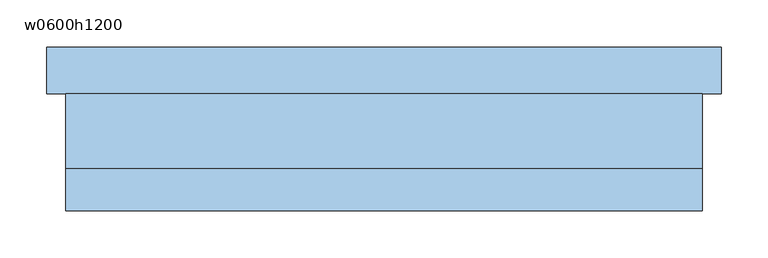
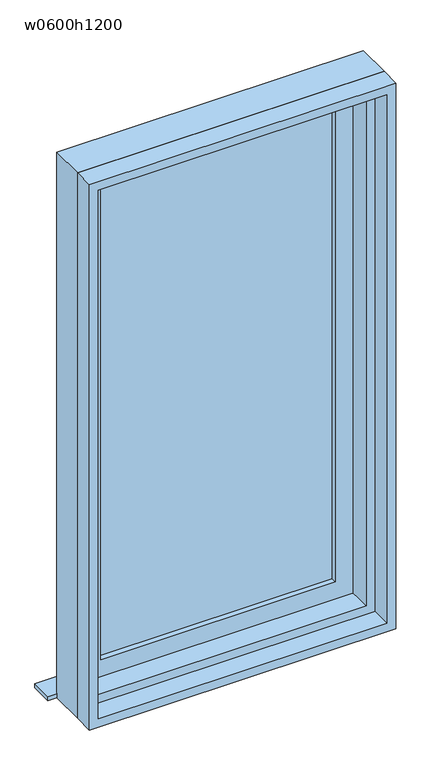
"""IFC4 building model written with IfcOpenShell, lengths in millimetres: window geometry, 縦すべり窓 : w0600h1200."""

import ifcopenshell
import ifcopenshell.guid

model = None  # the IFC model being written
_history = None  # IfcOwnerHistory: only IFC2X3 demands one
_inside = {}  # id of a spatial element -> (the spatial element, [elements in it])
_under = {}  # id of a project, library or spatial element -> (it, [spatial elements below it])
_declared = {}  # id of a project -> (the project, [libraries it declares])
_typed = {}  # id of a type object -> (the type object, [elements of that type])
_made_of = {}  # id of a material, layer set ... -> (it, [elements and type objects made of it])


def new_model(schema):
    """Start an empty IFC model of exactly this schema.

    Asked for "IFC4X3", IfcOpenShell would pick the latest addendum, in which some entities
    have other attributes; the version numbers below select the first issue.
    IFC2X3 requires an IfcOwnerHistory on every rooted entity: one is made here for all.
    """
    global model, _history
    if schema == "IFC4X3":
        model = ifcopenshell.file(schema_version=(4, 3, 0, 0))
    else:
        model = ifcopenshell.file(schema=schema)
    _inside.clear()
    _under.clear()
    _declared.clear()
    _typed.clear()
    _made_of.clear()
    _history = None
    if model.schema == "IFC2X3":
        org = make("IfcOrganization", Name="unknown")
        user = make(
            "IfcPersonAndOrganization",
            ThePerson=make("IfcPerson", FamilyName="unknown"),
            TheOrganization=org,
        )
        app = make(
            "IfcApplication",
            ApplicationDeveloper=org,
            Version="unknown",
            ApplicationFullName="unknown",
            ApplicationIdentifier="unknown",
        )
        _history = make(
            "IfcOwnerHistory",
            OwningUser=user,
            OwningApplication=app,
            ChangeAction="ADDED",
            CreationDate=0,
        )
    return model


def make(cls, **values):
    """One entity of the class cls with the attributes given. An attribute that is None is left unset."""
    return model.create_entity(
        cls, **{name: value for name, value in values.items() if value is not None}
    )


def rooted(cls, **values):
    """An entity with a GlobalId (a new one), such as an element, a storey or a relation."""
    return make(cls, GlobalId=ifcopenshell.guid.new(), OwnerHistory=_history, **values)


def si_unit(unit_type, name, prefix=None):
    """IfcSIUnit, for example si_unit("LENGTHUNIT", "METRE", prefix="MILLI")."""
    return make("IfcSIUnit", UnitType=unit_type, Prefix=prefix, Name=name)


def assignment(units):
    """IfcUnitAssignment: the units of a project."""
    return None if units is None else make("IfcUnitAssignment", Units=units)


def point(xyz):
    """IfcCartesianPoint."""
    return None if xyz is None else make("IfcCartesianPoint", Coordinates=xyz)


def direction(xyz):
    """IfcDirection."""
    return None if xyz is None else make("IfcDirection", DirectionRatios=xyz)


def frame(location, z_axis=None, x_axis=None):
    """IfcAxis2Placement3D, a coordinate frame: its origin and axes. An axis left out is left unset."""
    return make(
        "IfcAxis2Placement3D",
        Location=point(location),
        Axis=direction(z_axis),
        RefDirection=direction(x_axis),
    )


def origin():
    """The frame at (0, 0, 0) with its axes left unset."""
    return frame((0.0, 0.0, 0.0))


def place(relative_to, where):
    """IfcLocalPlacement: puts the frame where relative to a parent placement (None: the world)."""
    return make(
        "IfcLocalPlacement", PlacementRelTo=relative_to, RelativePlacement=where
    )


def context(
    kind, dimensions, precision=None, world=None, true_north=None, identifier=None
):
    """IfcGeometricRepresentationContext, for example the 3D "Model" context."""
    return make(
        "IfcGeometricRepresentationContext",
        ContextIdentifier=identifier,
        ContextType=kind,
        CoordinateSpaceDimension=dimensions,
        Precision=precision,
        WorldCoordinateSystem=world,
        TrueNorth=true_north,
    )


def project(units=None, contexts=None):
    """IfcProject with its units and contexts."""
    return rooted(
        "IfcProject",
        Name="project",
        RepresentationContexts=contexts,
        UnitsInContext=assignment(units),
    )


def spatial(cls, under=None, at=None, **own):
    """A site, building, storey or space (cls), placed at a placement, below another one or the project."""
    s = rooted(cls, ObjectPlacement=at, **own)
    if under is not None:
        _under.setdefault(under.id(), (under, []))[1].append(s)
    return s


def polyline(points):
    """IfcPolyline through the points."""
    return make("IfcPolyline", Points=[point(p) for p in points])


def outline(outer, holes=None, kind="AREA"):
    """IfcArbitraryClosedProfileDef: a profile drawn as a closed curve; with holes, ...WithVoids."""
    if holes is None:
        return make("IfcArbitraryClosedProfileDef", ProfileType=kind, OuterCurve=outer)
    return make(
        "IfcArbitraryProfileDefWithVoids",
        ProfileType=kind,
        OuterCurve=outer,
        InnerCurves=holes,
    )


def extrude(swept, where, along, depth):
    """IfcExtrudedAreaSolid: the profile swept, set in the frame where, extruded along a direction by depth."""
    return make(
        "IfcExtrudedAreaSolid",
        SweptArea=swept,
        Position=where,
        ExtrudedDirection=direction(along),
        Depth=depth,
    )


def shape(context_of_items, identifier, shape_type, items):
    """IfcShapeRepresentation: the items that make up one representation, for example the "Body"."""
    return make(
        "IfcShapeRepresentation",
        ContextOfItems=context_of_items,
        RepresentationIdentifier=identifier,
        RepresentationType=shape_type,
        Items=items,
    )


def source(mapping_origin, context_of_items, identifier, shape_type, items):
    """IfcRepresentationMap: a shape defined once, which mapped items show again and again."""
    return make(
        "IfcRepresentationMap",
        MappingOrigin=mapping_origin,
        MappedRepresentation=shape(context_of_items, identifier, shape_type, items),
    )


def transform(
    local_origin,
    x_axis=None,
    y_axis=None,
    z_axis=None,
    scale=None,
    scale2=None,
    scale3=None,
    uniform=True,
):
    """IfcCartesianTransformationOperator3D, or its non-uniform kind. x_axis, y_axis, z_axis: its Axis1, 2, 3."""
    if uniform:
        return make(
            "IfcCartesianTransformationOperator3D",
            Axis1=direction(x_axis),
            Axis2=direction(y_axis),
            LocalOrigin=point(local_origin),
            Scale=scale,
            Axis3=direction(z_axis),
        )
    return make(
        "IfcCartesianTransformationOperator3DnonUniform",
        Axis1=direction(x_axis),
        Axis2=direction(y_axis),
        LocalOrigin=point(local_origin),
        Scale=scale,
        Axis3=direction(z_axis),
        Scale2=scale2,
        Scale3=scale3,
    )


def mapped(mapping_source, mapping_target):
    """IfcMappedItem: shows the shape of a source again, moved by a transform."""
    return make(
        "IfcMappedItem", MappingSource=mapping_source, MappingTarget=mapping_target
    )


def made_of(thing, what):
    """Note that an element or type object is made of a material, layer set ...; save() writes the relation."""
    if what is not None:
        _made_of.setdefault(what.id(), (what, []))[1].append(thing)
    return thing


def element(
    cls,
    number,
    at=None,
    inside=None,
    cuts=None,
    type_object=None,
    material=None,
    context=None,
    identifier="Body",
    shape_type=None,
    held_by="IfcProductDefinitionShape",
    body=None,
    shapes=None,
    **own,
):
    """One element of the class cls, such as IfcWall. Its Tag is "e" and its number.

    at: its placement. inside: the storey or other place that contains it. cuts: it is an
    opening in that element (IfcRelVoidsElement). A single representation is given by context,
    identifier, shape_type and body (its items); several are given by shapes. held_by: the class
    of the entity that holds the representations. save() writes the other relations.
    """
    e = rooted(cls, Tag="e%d" % number, ObjectPlacement=at, **own)
    if body is not None:
        shapes = [shape(context, identifier, shape_type, body)]
    if shapes is not None:
        e.Representation = make(held_by, Representations=shapes)
    if inside is not None:
        _inside.setdefault(inside.id(), (inside, []))[1].append(e)
    if cuts is not None:
        rooted(
            "IfcRelVoidsElement", RelatingBuildingElement=cuts, RelatedOpeningElement=e
        )
    if type_object is not None:
        _typed.setdefault(type_object.id(), (type_object, []))[1].append(e)
    return made_of(e, material)


def aggregate(whole, parts):
    """IfcRelAggregates: a whole, such as a stair, and the parts it consists of."""
    return rooted("IfcRelAggregates", RelatingObject=whole, RelatedObjects=parts)


def save(model, path):
    """Write the relations noted so far, then the file.

    IfcRelAggregates (storeys below a building ...), IfcRelContainedInSpatialStructure (elements
    in a storey), IfcRelDefinesByType, IfcRelAssociatesMaterial and IfcRelDeclares: one each for
    every whole, place, type object, material and project.
    """
    for whole, parts in _under.values():
        aggregate(whole, parts)
    for where, things in _inside.values():
        rooted(
            "IfcRelContainedInSpatialStructure",
            RelatedElements=things,
            RelatingStructure=where,
        )
    for kind, things in _typed.values():
        rooted("IfcRelDefinesByType", RelatedObjects=things, RelatingType=kind)
    for what, things in _made_of.values():
        rooted("IfcRelAssociatesMaterial", RelatedObjects=things, RelatingMaterial=what)
    for by, libraries in _declared.values():
        rooted("IfcRelDeclares", RelatingContext=by, RelatedDefinitions=libraries)
    model.write(path)


def w0600h1200_d3eda8cc(model_context):
    return source(origin(), model_context, "Body", "SweptSolid", [
        extrude(outline(polyline([(260.0, 22.5), (-260.0, 22.5), (-260.0, 27.5), (260.0, 27.5), (260.0, 22.5)])), frame((0.0, 0.0, 840.0), z_axis=(0.0, 0.0, 1.0), x_axis=(1.0, 0.0, 0.0)), (0.0, 0.0, 1.0), 1120.0),
        extrude(outline(polyline([(2000.0, 300.0), (2000.0, -300.0), (800.0, -300.0), (800.0, 300.0), (2000.0, 300.0)]), holes=[polyline([(1960.0, -260.0), (1960.0, 260.0), (840.0, 260.0), (840.0, -260.0), (1960.0, -260.0)])]), frame((0.0, 10.0, 0.0), z_axis=(0.0, 1.0, 0.0), x_axis=(0.0, 0.0, 1.0)), (0.0, 0.0, 1.0), 30.0),
        extrude(outline(polyline([(360.0, 90.0), (360.0, 40.0), (-360.0, 40.0), (-360.0, 90.0), (360.0, 90.0)])), frame((0.0, 0.0, 760.0), z_axis=(0.0, 0.0, 1.0), x_axis=(1.0, 0.0, 0.0)), (0.0, 0.0, 1.0), 10.0),
        extrude(outline(polyline([(2040.0, 340.0), (2040.0, -340.0), (760.0, -340.0), (760.0, 340.0), (2040.0, 340.0)]), holes=[polyline([(780.0, -320.0), (2020.0, -320.0), (2020.0, 320.0), (780.0, 320.0), (780.0, -320.0)])]), frame((0.0, -85.0, 0.0), z_axis=(0.0, 1.0, 0.0), x_axis=(0.0, 0.0, 1.0)), (0.0, 0.0, 1.0), 45.0),
        extrude(outline(polyline([(2040.0, -340.0), (760.0, -340.0), (760.0, 340.0), (2040.0, 340.0), (2040.0, -340.0)]), holes=[polyline([(2000.0, 300.0), (800.0, 300.0), (800.0, -300.0), (2000.0, -300.0), (2000.0, 300.0)])]), frame((0.0, -40.0, 0.0), z_axis=(0.0, 1.0, 0.0), x_axis=(0.0, 0.0, 1.0)), (0.0, 0.0, 1.0), 80.0),
    ])


if __name__ == "__main__":
    model = new_model("IFC4")
    model_context = context("Model", 3, world=origin())
    ifc_project = project(units=[si_unit("LENGTHUNIT", "METRE", prefix="MILLI")], contexts=[model_context])
    site = spatial("IfcSite", under=ifc_project)
    building = spatial("IfcBuilding", under=site)
    placement = place(None, origin())
    w0600h1200_shape = w0600h1200_d3eda8cc(model_context)
    element("IfcWindow", 1, ObjectType="縦すべり窓 : w0600h1200", at=placement, inside=building, context=model_context, shape_type="MappedRepresentation", body=[
        mapped(w0600h1200_shape, transform((0.0, 0.0, 0.0), x_axis=(1.0, 0.0, 0.0), y_axis=(0.0, 1.0, 0.0), z_axis=(0.0, 0.0, 1.0))),
    ])
    save(model, "model.ifc")

# Revit data of these elements
# Type "縦すべり窓 : w0600h1200"
#   Construction Type Id = "GSP4R"
#   Analytic Construction = "1/8 インチ ピルキントン一重ガラス"
#   Type Mark = "86"
#   Operation = "シングルパネル"
#   Keynote = "08520.S3"
#   Visual Light Transmittance = 0.9
#   Solar Heat Gain Coefficient = 0.86
#   Heat Transfer Coefficient (U) = 6.7069 W/(m²·K)
#   Height = 1200 mm
#   既定の腰高 = 800 mm
#   Width = 600 mm
#   額縁見附 = 20 mm
#   額縁ちり = 10 mm
#   サッシ見附 = 40 mm
#   サッシの幅 = 80 mm
#   サッシ額縁 [instance default] = none
#   サッシ本体 [instance default] = none
#   サッシガラス [instance default] = ガラス - 透明
#   Wall Closure = (empty or 0)
#   Type Comments = ""
#   Assembly Code = ""
# Element 1 (IfcWindow, "縦すべり窓 : w0600h1200")
#   Materials on its faces: "ガラス - 透明"
# Materials
#   "ガラス - 透明": class "ガラス", colour RGB 0 128 192, transparency 0.9, Cost = 0
